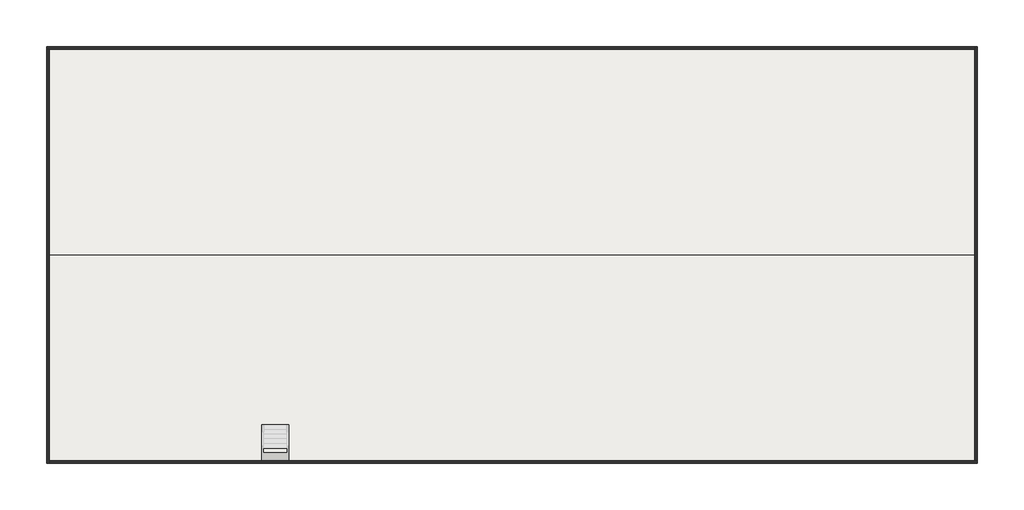
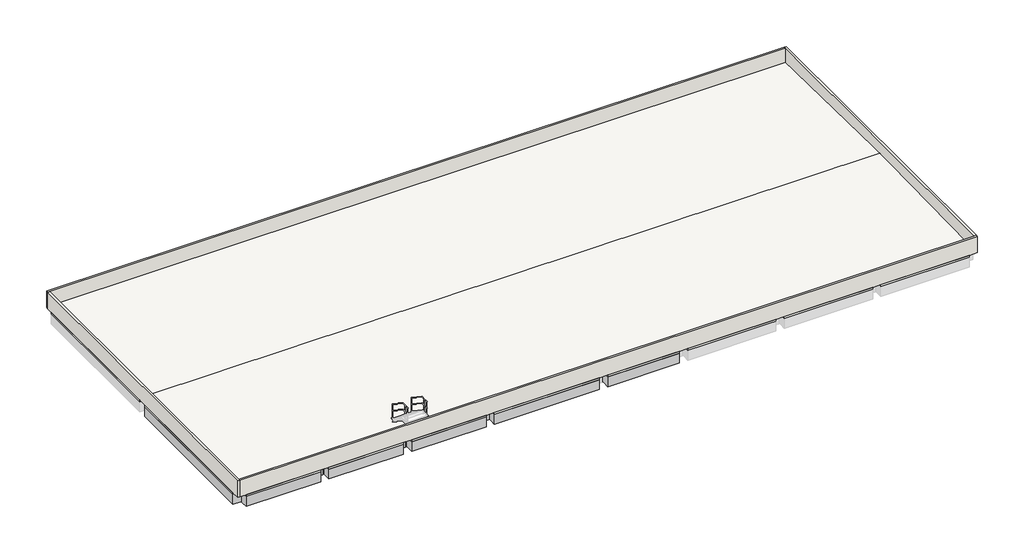
# One storey, part 1 of 3: 16 beams, 4 walls, 1 roof, 1 slab.
# Revit data of these elements (continued)
# Type "RC Beam_Rectangular : H_SB_AR_S16_B400xH900_RB1" (continued)
#   Length [instance default] = 1524 mm
#   b = 400 mm
#   h = 900 mm
#   hec_material3 [instance default] = none
#   hec_material2 [instance default] = none
#   hec_material1 [instance default] = none
#   Structural Material [instance default] = none
#   Assembly Code = ""
# Type "RC Beam_Rectangular : H_SB_AR_S16_B600xH900_RB3"
#   H_Q'ty Cal Type Tag = "CE-Q1"
#   중앙부 하부근 = ""
#   중앙부 상부근 = ""
#   중앙부 보조근 = ""
#   중앙부 늑근 = ""
#   외단부 하부근 = ""
#   외단부 상부근 = ""
#   외단부 보조근 = ""
#   외단부 늑근 = ""
#   부호 = "TG3"
#   내단부 하부근 = ""
#   내단부 상부근 = ""
#   내단부 보조근 = ""
#   내단부 늑근 = ""
#   ALL 하부근 = "3-D20"
#   ALL 상부근 = "3-D20"
#   ALL 보조근 = ""
#   ALL 늑근 = "2-D10 @120"
#   Width = 600 mm
#   Height = 900 mm
#   Length [instance default] = 1524 mm
#   b = 600 mm
#   h = 900 mm
#   hec_material3 [instance default] = none
#   hec_material2 [instance default] = none
#   hec_material1 [instance default] = none
#   Structural Material [instance default] = none
#   Assembly Code = ""
# Type "H_RF_AR_B06_Mortar(Slope)_XPS_Memb_T50+120"
#   H_Q'ty Cal Type Tag = "RF-Q1"
#   H_WM Code_1 = "A04AQ086-00004 |  | M3 | Finishing Work | Roof Work | Roof Screed | Bed Mortar Screed | w/o Welded Wire Fabric | 30mm≤Min. THK<50mm | Min. THK=(  )mm, Slope=(  ) | A04AQ086-00004 Finishing Work Roof Work Roof Screed Bed Mortar Screed     w/o Welded Wire Fabric  30mm≤Min. THK<50mm | Min. THK=( 30 )mm, Slope=( 1% )"
#   H_WM Code_2 = "A04AQ038-00001 |  | M2 | Finishing Work | Roof Work | Welded Wire Fabric | DIA≤6mm | Mesh Size=DIA(  )mm x (  )mm x (  )mm | A04AQ038-00001 Finishing Work Roof Work Welded Wire Fabric        DIA≤6mm | Mesh Size=DIA( #8 )mm x ( 150 )mm x (150  )mm"
#   H_WM Code_3 = "A04AQ012-00001 |  | M2 | Finishing Work | Roof Work | PE Sheet (Vapor Barrier) |  | THK=(  )mm | A04AQ012-00001 Finishing Work Roof Work PE Sheet (Vapor Barrier)         | THK=( 0.1 )mm, 2ply"
#   H_WM Code_4 = "A04AQ088-00004 |  | M2 | Finishing Work | Roof Work | Roof Insulation | Rigid Extruded Polystyrene Foam Insulation |  | 100mm≤THK | THK=(  )mm | A04AQ088-00004 Finishing Work Roof Work Roof Insulation Rigid Extruded Polystyrene Foam Insulation       100mm≤THK | THK=( 120 )mm"
#   H_WM Code_5 = "A04AQ310-00001 |  | M2 | Finishing Work | Roof Work | Waterproofing Membrane | EPDM(or Equivalent) | w/ Accessories | THK=(  )mm | A04AQ310-00001 Finishing Work Roof Work Waterproofing Membrane EPDM(or Equivalent)     w/ Accessories   |"
#   Layers, outside or top first: 1.5 mm "Roofing - EPDM Membrane" (function 4); 120 mm "00_Insulation_Rigid_hec" (function 3); 50 mm "Slab, Screed" (function 1)
# Type "H_FL_AR_S17_Roof RC Slab_T150"
#   Keynote = ""
#   Type Comments = ""
#   Description = ""
#   H_Q'ty Cal Type Tag = "FL-Q1"
#   H_WM Code_1 = "A03AF032-00007 |  | M3 | Concrete Work | Superstructure Work | Structural Concrete | Cement Type-1 | 25MPa < F'c (Cylinder Strength) ≤ 30MPa |  |  |  | A03AF032-00007 Concrete Work Superstructure Work Structural Concrete  Cement Type-1 25MPa < F'c (Cylinder Strength) ≤ 30MPa      |  F'c (Cylinder Strength) = 24MPa"
#   H_WM Code_2 = "A03AF037-00003 |  | TON | Concrete Work | Superstructure Work | Rebar Work | Deformed Bar (Non-Coat.) | 300MPa<Fy≤400MPa |  |  |  | A03AF037-00003 Concrete Work Superstructure Work Rebar Work Deformed Bar (Non-Coat.)  300MPa<Fy≤400MPa      | ASTM A615 GRADE 60 (Fy=420MPa)"
#   H_WM Code_3 = "A03AF036-00001 |  | M2 | Concrete Work | Superstructure Work | Form Work (1 time in use) | Flat Form | Dressed Lumber, Plywood or Steel Form(Wood Planks are not Allowed) incl. Chamfer |  |  | A03AF036-00001 Concrete Work Superstructure Work Form Work (1 time in use) Flat Form     Dressed Lumber, Plywood or Steel Form(Wood Planks are not Allowed) incl. Chamfer   |"
#   Function = 1
#   Layers, outside or top first: 150 mm "Concrete - Cast-in-Place Concrete - 35 MPa" (function 1)
# Type "H_WA_AR_B02_Ext Wall_RC T150"
#   Type Comments = ""
#   H_Q'ty Cal Type Tag = "WA-Q1"
#   H_WM Code_1 = "A03AD032-00010 |  | M3 | Concrete Work | Substructure Work | Structural Concrete | Cement Type-1 | 20MPa < F'c (Cylinder Strength) ≤ 25MPa |  |  |  | A03AD032-00010 Concrete Work Substructure Work Structural Concrete  Cement Type-1 20MPa < F'c (Cylinder Strength) ≤ 25MPa      | ASTM C150 Type I or Type IA \nF'c (Cylinder Strength) = 28MPa"
#   H_WM Code_2 = "A03AD037-00002 |  | TON | Concrete Work | Substructure Work | Rebar Work | Deformed Bar (Non-Coat.) | 400MPa<Fy≤470MPa |  |  |  | A03AD037-00002 Concrete Work Substructure Work Rebar Work Deformed Bar (Non-Coat.)  400MPa<Fy≤470MPa      | ASTM A615 GRADE 60 (Fy=420MPa)"
#   H_WM Code_3 = "A03AD036-00001 |  | M2 | Concrete Work | Substructure Work | Form Work (1 time in use) | Flat Form | Dressed Lumber, Plywood or Steel Form(Wood Planks are not Allowed) incl. Chamfer |  |  | A03AD036-00001 Concrete Work Substructure Work Form Work (1 time in use) Flat Form     Dressed Lumber, Plywood or Steel Form(Wood Planks are not Allowed) incl. Chamfer   |"
#   Layers, outside or top first: 150 mm "Concrete - Cast-in-Place Concrete - 35 MPa" (function 1)
# Elements 1, 2, 3 (IfcBeam, "RC Beam_Rectangular : H_SB_AR_S16_B600xH900_RG4")
#   Comments = ""
#   hec_material3 = none
#   hec_material2 = none
#   hec_material1 = none
#   Structural Material = Concrete - Cast-in-Place Concrete - 35 MPa
#   Phase Created = New Construction
#   Materials on its faces: "Concrete - Cast-in-Place Concrete - 35 MPa"
# Elements 4, 5, 6, 7, 8 (IfcBeam, "RC Beam_Rectangular : H_SB_AR_S16_B600xH900_RG9")
#   Comments = ""
#   hec_material3 = none
#   hec_material2 = none
#   hec_material1 = none
#   Structural Material = Concrete - Cast-in-Place Concrete - 35 MPa
#   Phase Created = New Construction
#   Materials on its faces: "Concrete - Cast-in-Place Concrete - 35 MPa"
# Element 9 (IfcBeam, "RC Beam_Rectangular : H_SB_AR_S16_B600xH900_RG6")
#   Comments = ""
#   hec_material3 = none
#   hec_material2 = none
#   hec_material1 = none
#   Structural Material = Concrete - Cast-in-Place Concrete - 35 MPa
#   Phase Created = New Construction
#   Materials on its faces: "Concrete - Cast-in-Place Concrete - 35 MPa"
# Elements 10, 11 (IfcBeam, "RC Beam_Rectangular : H_SB_AR_S16_B400xH900_RG1")
#   Comments = ""
#   hec_material3 = none
#   hec_material2 = none
#   hec_material1 = none
#   Structural Material = Concrete - Cast-in-Place Concrete - 35 MPa
#   Phase Created = New Construction
#   Materials on its faces: "Concrete - Cast-in-Place Concrete - 35 MPa"
# Element 12 (IfcBeam, "RC Beam_Rectangular : H_SB_AR_S16_B600xH900_RG1A")
#   Comments = ""
#   hec_material3 = none
#   hec_material2 = none
#   hec_material1 = none
#   Structural Material = Concrete - Cast-in-Place Concrete - 35 MPa
#   Phase Created = New Construction
#   Materials on its faces: "Concrete - Cast-in-Place Concrete - 35 MPa"
# Elements 13, 14, 15 (IfcBeam, "RC Beam_Rectangular : H_SB_AR_S16_B400xH900_RB1")
#   hec_material3 = none
#   hec_material2 = none
#   hec_material1 = none
#   Structural Material = Concrete - Cast-in-Place Concrete - 35 MPa
#   Phase Created = New Construction
#   Materials on its faces: "Concrete - Cast-in-Place Concrete - 35 MPa"
# Element 16 (IfcBeam, "RC Beam_Rectangular : H_SB_AR_S16_B600xH900_RB3")
#   hec_material3 = none
#   hec_material2 = none
#   hec_material1 = none
#   Structural Material = Concrete - Cast-in-Place Concrete - 35 MPa
#   Phase Created = New Construction
#   Materials on its faces: "Concrete - Cast-in-Place Concrete - 35 MPa"
# Element 17 (IfcRoof, "H_RF_AR_B06_Mortar(Slope)_XPS_Memb_T50+120")
#   H_Roof Style Name = "Concrete Slab(Slope)+Insulation+Protection Concrete+Waterproofing"
#   H_Roof_Base Material = "Concrete Slab"
#   H_Roof_Finish-1 = "Liquid Waterproofing"
#   H_Roof_Finish-2 = "Rigid Extruded Polystyrene Foam Insulation(XPS)"
#   H_Roof_Finish-3 = "Welded Wire Fabric"
#   H_Roof_Finish-4 = "Protective Concrete w/ Steel Trowel Finish"
#   H_Roof_Finish-5 = "스카이패널 건식복합방수"
#   H_Roof_Style Remark = "* 스카이패널 건식복합방수 : WM 없음"
#   built-in parameter 1001705 = 25.1688 (stored number, unit not read)
#   built-in parameter 1001710 = 33615
#   H_Roof Style No = RF41
#   Phase Created = New Construction
#   Materials on its faces: "Slab, Screed", "Roofing - EPDM Membrane"
# Element 18 (IfcSlab, "H_FL_AR_S17_Roof RC Slab_T150")
#   Comments = ""
#   TMP_Element Name = "SS2"
#   Height Offset From Level = 0 mm
#   built-in parameter 1001954 = 1
#   Phase Created = New Construction
#   Materials on its faces: "Concrete - Cast-in-Place Concrete - 35 MPa"
# Elements 19, 20, 21, 22 (IfcWall, "H_WA_AR_B02_Ext Wall_RC T150")
#   Top Offset = 0 mm
#   Base Offset = 0 mm
#   wall height = 1250 mm
#   Phase Created = New Construction
#   Base Constraint = TOC
#   Top Constraint = TOP
#   Materials on its faces: "Concrete - Cast-in-Place Concrete - 35 MPa"
# Materials
#   "Roofing - EPDM Membrane": class "Plastic", colour RGB 127 127 127, transparency 0, Description = "Exterior finish, roofing"
#   "00_Insulation_Rigid_hec": class "Insulation", colour RGB 255 255 217, transparency 0, Description = "Insulation(Rigid)", Cost = 0
#   "Slab, Screed": class "Concrete", colour RGB 120 120 120, transparency 0, Description = "Concrete slab topping", Cost = 0
#   "Concrete - Cast-in-Place Concrete - 35 MPa": class "Concrete", colour RGB 192 192 192, transparency 0, Description = "ACRYLIC EMULSION PAINT ON THK.13 CEMENT PLASTER", Cost = 0
